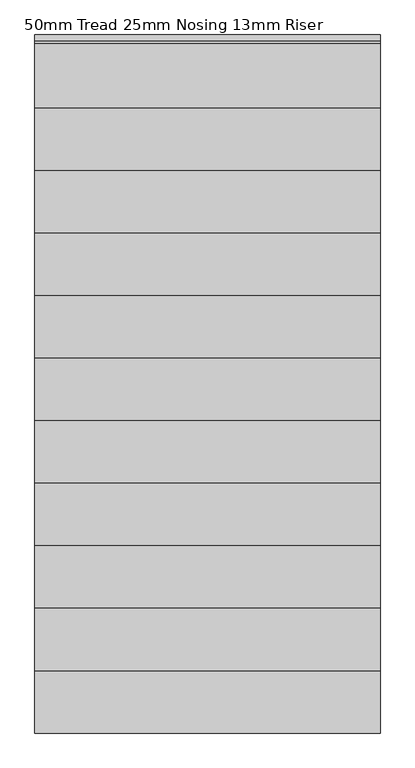
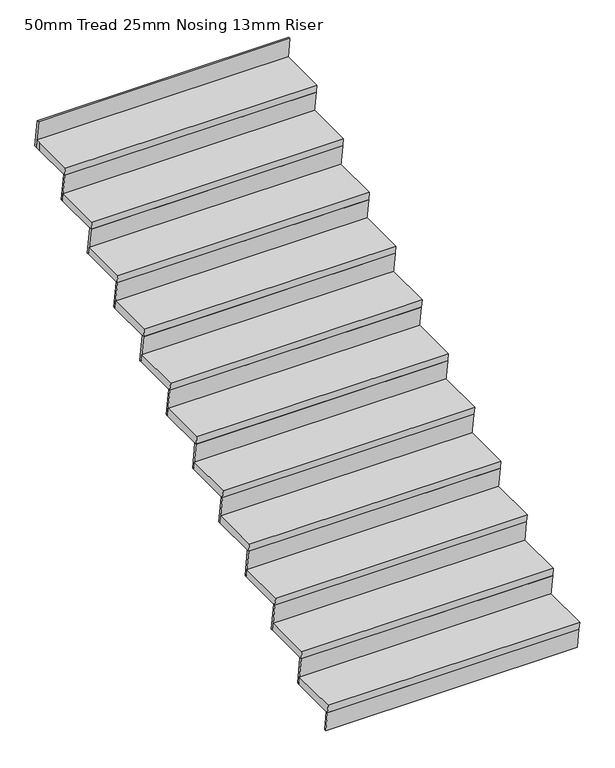
"""IFC4 building model written with IfcOpenShell, lengths in millimetres: stair flight geometry, 50mm Tread 25mm Nosing 13mm Riser."""

from ifc_helpers import new_model, si_unit, origin, place, context, project, spatial, faceted_brep, source, transform, mapped, element, save


def stair_flight_50mm_tread_25mm_nosing_13mm_riser_1a7390ad(model_context):
    return source(origin(), model_context, "Body", "Brep", [
        faceted_brep([(-499.4393676, 4584.7509075, 3676.4705882), (-499.4393676, 4591.8342409, 3626.4705882), (-2019.4393676, 4591.8342409, 3626.4705882), (-2019.4393676, 4584.7509075, 3676.4705882), (-2019.4393676, 4284.7509075, 3676.4705882), (-499.4393676, 4284.7509075, 3676.4705882), (-499.4393676, 4291.8342409, 3626.4705882), (-2019.4393676, 4291.8342409, 3626.4705882)], [[[0, 1, 2, 3]], [[3, 4, 5, 0]], [[2, 1, 6, 7]], [[4, 3, 2, 7]], [[0, 5, 6, 1]], [[5, 4, 7, 6]]]),
        faceted_brep([(-499.4393676, 4291.8342409, 3626.4705882), (-499.4393676, 4309.7509075, 3500.0), (-499.4393676, 4322.3757185, 3500.0), (-499.4393676, 4304.4590518, 3626.4705882), (-2019.4393676, 4291.8342409, 3626.4705882), (-2019.4393676, 4304.4590518, 3626.4705882), (-2019.4393676, 4322.3757185, 3500.0), (-2019.4393676, 4309.7509075, 3500.0)], [[[0, 1, 2, 3]], [[4, 5, 6, 7]], [[1, 0, 4, 7]], [[2, 1, 7, 6]], [[3, 2, 6, 5]], [[0, 3, 5, 4]]]),
        faceted_brep([(-499.4393676, 4566.8342409, 3802.9411765), (-499.4393676, 4591.8342409, 3626.4705882), (-499.4393676, 4604.4590518, 3626.4705882), (-499.4393676, 4579.4590518, 3802.9411765), (-2019.4393676, 4566.8342409, 3802.9411765), (-2019.4393676, 4579.4590518, 3802.9411765), (-2019.4393676, 4604.4590518, 3626.4705882), (-2019.4393676, 4591.8342409, 3626.4705882)], [[[0, 1, 2, 3]], [[4, 5, 6, 7]], [[1, 0, 4, 7]], [[2, 1, 7, 6]], [[3, 2, 6, 5]], [[0, 3, 5, 4]]]),
        faceted_brep([(-2019.4393676, 4859.7509075, 3852.9411765), (-2019.4393676, 4559.7509075, 3852.9411765), (-499.4393676, 4559.7509075, 3852.9411765), (-499.4393676, 4859.7509075, 3852.9411765), (-2019.4393676, 4866.8342409, 3802.9411765), (-499.4393676, 4866.8342409, 3802.9411765), (-499.4393676, 4566.8342409, 3802.9411765), (-2019.4393676, 4566.8342409, 3802.9411765)], [[[0, 1, 2, 3]], [[4, 5, 6, 7]], [[1, 0, 4, 7]], [[3, 2, 6, 5]], [[3, 5, 4, 0]], [[2, 1, 7, 6]]]),
        faceted_brep([(-499.4393676, 4841.8342409, 3979.4117647), (-499.4393676, 4866.8342409, 3802.9411765), (-499.4393676, 4879.4590518, 3802.9411765), (-499.4393676, 4854.4590518, 3979.4117647), (-2019.4393676, 4841.8342409, 3979.4117647), (-2019.4393676, 4854.4590518, 3979.4117647), (-2019.4393676, 4879.4590518, 3802.9411765), (-2019.4393676, 4866.8342409, 3802.9411765)], [[[0, 1, 2, 3]], [[4, 5, 6, 7]], [[1, 0, 4, 7]], [[2, 1, 7, 6]], [[3, 2, 6, 5]], [[0, 3, 5, 4]]]),
        faceted_brep([(-2019.4393676, 5134.7509075, 4029.4117647), (-2019.4393676, 4834.7509075, 4029.4117647), (-499.4393676, 4834.7509075, 4029.4117647), (-499.4393676, 5134.7509075, 4029.4117647), (-2019.4393676, 5141.8342409, 3979.4117647), (-499.4393676, 5141.8342409, 3979.4117647), (-499.4393676, 4841.8342409, 3979.4117647), (-2019.4393676, 4841.8342409, 3979.4117647)], [[[0, 1, 2, 3]], [[4, 5, 6, 7]], [[1, 0, 4, 7]], [[3, 2, 6, 5]], [[3, 5, 4, 0]], [[2, 1, 7, 6]]]),
        faceted_brep([(-499.4393676, 5116.8342409, 4155.8823529), (-499.4393676, 5141.8342409, 3979.4117647), (-499.4393676, 5154.4590518, 3979.4117647), (-499.4393676, 5129.4590518, 4155.8823529), (-2019.4393676, 5116.8342409, 4155.8823529), (-2019.4393676, 5129.4590518, 4155.8823529), (-2019.4393676, 5154.4590518, 3979.4117647), (-2019.4393676, 5141.8342409, 3979.4117647)], [[[0, 1, 2, 3]], [[4, 5, 6, 7]], [[1, 0, 4, 7]], [[2, 1, 7, 6]], [[3, 2, 6, 5]], [[0, 3, 5, 4]]]),
        faceted_brep([(-2019.4393676, 5409.7509075, 4205.8823529), (-2019.4393676, 5109.7509075, 4205.8823529), (-499.4393676, 5109.7509075, 4205.8823529), (-499.4393676, 5409.7509075, 4205.8823529), (-2019.4393676, 5416.8342409, 4155.8823529), (-499.4393676, 5416.8342409, 4155.8823529), (-499.4393676, 5116.8342409, 4155.8823529), (-2019.4393676, 5116.8342409, 4155.8823529)], [[[0, 1, 2, 3]], [[4, 5, 6, 7]], [[1, 0, 4, 7]], [[3, 2, 6, 5]], [[3, 5, 4, 0]], [[2, 1, 7, 6]]]),
        faceted_brep([(-499.4393676, 5391.8342409, 4332.3529412), (-499.4393676, 5416.8342409, 4155.8823529), (-499.4393676, 5429.4590518, 4155.8823529), (-499.4393676, 5404.4590518, 4332.3529412), (-2019.4393676, 5391.8342409, 4332.3529412), (-2019.4393676, 5404.4590518, 4332.3529412), (-2019.4393676, 5429.4590518, 4155.8823529), (-2019.4393676, 5416.8342409, 4155.8823529)], [[[0, 1, 2, 3]], [[4, 5, 6, 7]], [[1, 0, 4, 7]], [[2, 1, 7, 6]], [[3, 2, 6, 5]], [[0, 3, 5, 4]]]),
        faceted_brep([(-2019.4393676, 5684.7509075, 4382.3529412), (-2019.4393676, 5384.7509075, 4382.3529412), (-499.4393676, 5384.7509075, 4382.3529412), (-499.4393676, 5684.7509075, 4382.3529412), (-2019.4393676, 5691.8342409, 4332.3529412), (-499.4393676, 5691.8342409, 4332.3529412), (-499.4393676, 5391.8342409, 4332.3529412), (-2019.4393676, 5391.8342409, 4332.3529412)], [[[0, 1, 2, 3]], [[4, 5, 6, 7]], [[1, 0, 4, 7]], [[3, 2, 6, 5]], [[3, 5, 4, 0]], [[2, 1, 7, 6]]]),
        faceted_brep([(-499.4393676, 5666.8342409, 4508.8235294), (-499.4393676, 5691.8342409, 4332.3529412), (-499.4393676, 5704.4590518, 4332.3529412), (-499.4393676, 5679.4590518, 4508.8235294), (-2019.4393676, 5666.8342409, 4508.8235294), (-2019.4393676, 5679.4590518, 4508.8235294), (-2019.4393676, 5704.4590518, 4332.3529412), (-2019.4393676, 5691.8342409, 4332.3529412)], [[[0, 1, 2, 3]], [[4, 5, 6, 7]], [[1, 0, 4, 7]], [[2, 1, 7, 6]], [[3, 2, 6, 5]], [[0, 3, 5, 4]]]),
        faceted_brep([(-2019.4393676, 5959.7509075, 4558.8235294), (-2019.4393676, 5659.7509075, 4558.8235294), (-499.4393676, 5659.7509075, 4558.8235294), (-499.4393676, 5959.7509075, 4558.8235294), (-2019.4393676, 5966.8342409, 4508.8235294), (-499.4393676, 5966.8342409, 4508.8235294), (-499.4393676, 5666.8342409, 4508.8235294), (-2019.4393676, 5666.8342409, 4508.8235294)], [[[0, 1, 2, 3]], [[4, 5, 6, 7]], [[1, 0, 4, 7]], [[3, 2, 6, 5]], [[3, 5, 4, 0]], [[2, 1, 7, 6]]]),
        faceted_brep([(-499.4393676, 5941.8342409, 4685.2941176), (-499.4393676, 5966.8342409, 4508.8235294), (-499.4393676, 5979.4590518, 4508.8235294), (-499.4393676, 5954.4590518, 4685.2941176), (-2019.4393676, 5941.8342409, 4685.2941176), (-2019.4393676, 5954.4590518, 4685.2941176), (-2019.4393676, 5979.4590518, 4508.8235294), (-2019.4393676, 5966.8342409, 4508.8235294)], [[[0, 1, 2, 3]], [[4, 5, 6, 7]], [[1, 0, 4, 7]], [[2, 1, 7, 6]], [[3, 2, 6, 5]], [[0, 3, 5, 4]]]),
        faceted_brep([(-2019.4393676, 6234.7509075, 4735.2941176), (-2019.4393676, 5934.7509075, 4735.2941176), (-499.4393676, 5934.7509075, 4735.2941176), (-499.4393676, 6234.7509075, 4735.2941176), (-2019.4393676, 6241.8342409, 4685.2941176), (-499.4393676, 6241.8342409, 4685.2941176), (-499.4393676, 5941.8342409, 4685.2941176), (-2019.4393676, 5941.8342409, 4685.2941176)], [[[0, 1, 2, 3]], [[4, 5, 6, 7]], [[1, 0, 4, 7]], [[3, 2, 6, 5]], [[3, 5, 4, 0]], [[2, 1, 7, 6]]]),
        faceted_brep([(-499.4393676, 6216.8342409, 4861.7647059), (-499.4393676, 6241.8342409, 4685.2941176), (-499.4393676, 6254.4590518, 4685.2941176), (-499.4393676, 6229.4590518, 4861.7647059), (-2019.4393676, 6216.8342409, 4861.7647059), (-2019.4393676, 6229.4590518, 4861.7647059), (-2019.4393676, 6254.4590518, 4685.2941176), (-2019.4393676, 6241.8342409, 4685.2941176)], [[[0, 1, 2, 3]], [[4, 5, 6, 7]], [[1, 0, 4, 7]], [[2, 1, 7, 6]], [[3, 2, 6, 5]], [[0, 3, 5, 4]]]),
        faceted_brep([(-2019.4393676, 6509.7509075, 4911.7647059), (-2019.4393676, 6209.7509075, 4911.7647059), (-499.4393676, 6209.7509075, 4911.7647059), (-499.4393676, 6509.7509075, 4911.7647059), (-2019.4393676, 6516.8342409, 4861.7647059), (-499.4393676, 6516.8342409, 4861.7647059), (-499.4393676, 6216.8342409, 4861.7647059), (-2019.4393676, 6216.8342409, 4861.7647059)], [[[0, 1, 2, 3]], [[4, 5, 6, 7]], [[1, 0, 4, 7]], [[3, 2, 6, 5]], [[3, 5, 4, 0]], [[2, 1, 7, 6]]]),
        faceted_brep([(-499.4393676, 6491.8342409, 5038.2352941), (-499.4393676, 6516.8342409, 4861.7647059), (-499.4393676, 6529.4590518, 4861.7647059), (-499.4393676, 6504.4590518, 5038.2352941), (-2019.4393676, 6491.8342409, 5038.2352941), (-2019.4393676, 6504.4590518, 5038.2352941), (-2019.4393676, 6529.4590518, 4861.7647059), (-2019.4393676, 6516.8342409, 4861.7647059)], [[[0, 1, 2, 3]], [[4, 5, 6, 7]], [[1, 0, 4, 7]], [[2, 1, 7, 6]], [[3, 2, 6, 5]], [[0, 3, 5, 4]]]),
        faceted_brep([(-2019.4393676, 6784.7509075, 5088.2352941), (-2019.4393676, 6484.7509075, 5088.2352941), (-499.4393676, 6484.7509075, 5088.2352941), (-499.4393676, 6784.7509075, 5088.2352941), (-2019.4393676, 6791.8342409, 5038.2352941), (-499.4393676, 6791.8342409, 5038.2352941), (-499.4393676, 6491.8342409, 5038.2352941), (-2019.4393676, 6491.8342409, 5038.2352941)], [[[0, 1, 2, 3]], [[4, 5, 6, 7]], [[1, 0, 4, 7]], [[3, 2, 6, 5]], [[3, 5, 4, 0]], [[2, 1, 7, 6]]]),
        faceted_brep([(-499.4393676, 6766.8342409, 5214.7058824), (-499.4393676, 6791.8342409, 5038.2352941), (-499.4393676, 6804.4590518, 5038.2352941), (-499.4393676, 6779.4590518, 5214.7058824), (-2019.4393676, 6766.8342409, 5214.7058824), (-2019.4393676, 6779.4590518, 5214.7058824), (-2019.4393676, 6804.4590518, 5038.2352941), (-2019.4393676, 6791.8342409, 5038.2352941)], [[[0, 1, 2, 3]], [[4, 5, 6, 7]], [[1, 0, 4, 7]], [[2, 1, 7, 6]], [[3, 2, 6, 5]], [[0, 3, 5, 4]]]),
        faceted_brep([(-2019.4393676, 7059.7509075, 5264.7058824), (-2019.4393676, 6759.7509075, 5264.7058824), (-499.4393676, 6759.7509075, 5264.7058824), (-499.4393676, 7059.7509075, 5264.7058824), (-2019.4393676, 7066.8342409, 5214.7058824), (-499.4393676, 7066.8342409, 5214.7058824), (-499.4393676, 6766.8342409, 5214.7058824), (-2019.4393676, 6766.8342409, 5214.7058824)], [[[0, 1, 2, 3]], [[4, 5, 6, 7]], [[1, 0, 4, 7]], [[3, 2, 6, 5]], [[3, 5, 4, 0]], [[2, 1, 7, 6]]]),
        faceted_brep([(-499.4393676, 7316.8342409, 5567.6470588), (-499.4393676, 7341.8342409, 5391.1764706), (-499.4393676, 7354.4590518, 5391.1764706), (-499.4393676, 7329.4590518, 5567.6470588), (-2019.4393676, 7316.8342409, 5567.6470588), (-2019.4393676, 7329.4590518, 5567.6470588), (-2019.4393676, 7354.4590518, 5391.1764706), (-2019.4393676, 7341.8342409, 5391.1764706)], [[[0, 1, 2, 3]], [[4, 5, 6, 7]], [[1, 0, 4, 7]], [[2, 1, 7, 6]], [[3, 2, 6, 5]], [[0, 3, 5, 4]]]),
        faceted_brep([(-499.4393676, 7041.8342409, 5391.1764706), (-499.4393676, 7066.8342409, 5214.7058824), (-499.4393676, 7079.4590518, 5214.7058824), (-499.4393676, 7054.4590518, 5391.1764706), (-2019.4393676, 7041.8342409, 5391.1764706), (-2019.4393676, 7054.4590518, 5391.1764706), (-2019.4393676, 7079.4590518, 5214.7058824), (-2019.4393676, 7066.8342409, 5214.7058824)], [[[0, 1, 2, 3]], [[4, 5, 6, 7]], [[1, 0, 4, 7]], [[2, 1, 7, 6]], [[3, 2, 6, 5]], [[0, 3, 5, 4]]]),
        faceted_brep([(-2019.4393676, 7334.7509075, 5441.1764706), (-2019.4393676, 7309.7509075, 5441.1764706), (-2019.4393676, 7034.7509075, 5441.1764706), (-499.4393676, 7034.7509075, 5441.1764706), (-499.4393676, 7334.7509075, 5441.1764706), (-2019.4393676, 7341.8342409, 5391.1764706), (-499.4393676, 7341.8342409, 5391.1764706), (-499.4393676, 7041.8342409, 5391.1764706), (-2019.4393676, 7041.8342409, 5391.1764706), (-2019.4393676, 7309.7509075, 5391.1764706)], [[[0, 1, 2, 3, 4]], [[5, 6, 7, 8, 9]], [[1, 0, 5, 9]], [[2, 1, 9, 8]], [[4, 3, 7, 6]], [[4, 6, 5, 0]], [[3, 2, 8, 7]]]),
    ])


if __name__ == "__main__":
    model = new_model("IFC4")
    model_context = context("Model", 3, world=origin())
    ifc_project = project(units=[si_unit("LENGTHUNIT", "METRE", prefix="MILLI")], contexts=[model_context])
    site = spatial("IfcSite", under=ifc_project)
    building = spatial("IfcBuilding", under=site)
    placement = place(None, origin())
    stair_flight_50mm_tread_25mm_nosing_13mm_riser_shape = stair_flight_50mm_tread_25mm_nosing_13mm_riser_1a7390ad(model_context)
    element("IfcStairFlight", 1, ObjectType="50mm Tread 25mm Nosing 13mm Riser", at=placement, inside=building, context=model_context, shape_type="MappedRepresentation", body=[
        mapped(stair_flight_50mm_tread_25mm_nosing_13mm_riser_shape, transform((0.0, 0.0, 0.0), x_axis=(1.0, 0.0, 0.0), y_axis=(0.0, 1.0, 0.0), z_axis=(0.0, 0.0, 1.0))),
    ])
    save(model, "model.ifc")
